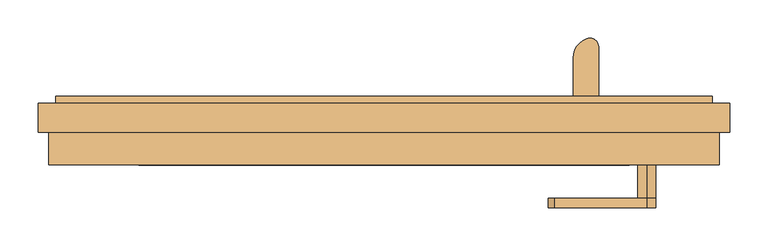
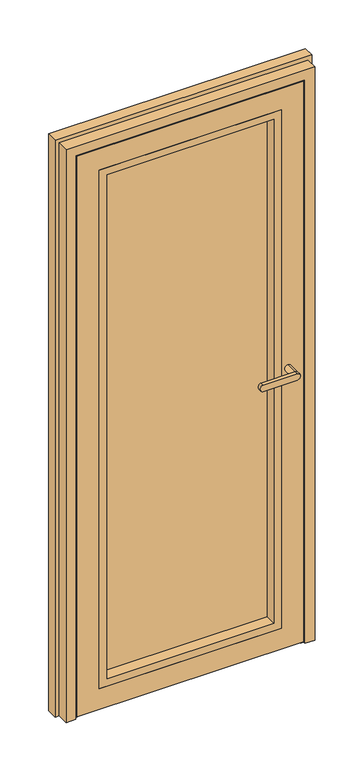
"""IFC4 building model written with IfcOpenShell, lengths in millimetres: door geometry, Schueco_FWS_ADS-90-SI_inw_Family-01 : FWS SI insert unit."""

from ifc_helpers import new_model, si_unit, point, frame, frame_2d, origin, place, context, project, spatial, polyline, circle_curve, ellipse_curve, trimmed, segment, composite_curve, outline, extrude, faceted_brep, source, transform, mapped, element, save
from ifc_brep_helpers import plane_surface, cylinder_surface, extruded_surface, advanced_brep


def door_b40c46e4(model_context):
    return source(origin(), model_context, "Body", "SolidModel", [
        extrude(outline(composite_curve([segment(polyline([(248.3327372, 8.9997177), (248.3327372, 59.1618682)]), True, "CONTINUOUS"), segment(trimmed(circle_curve(frame_2d((275.5111549, 59.1618682)), 27.1784177), [point((248.3327372, 59.1618682))], [point((265.9740593, 84.6120194))], False, "CARTESIAN"), True, "CONTINUOUS"), segment(trimmed(circle_curve(frame_2d((270.0515602, 73.7310321)), 11.6198924), [point((265.9740593, 84.6120194))], [point((281.6714526, 73.7310321))], False, "CARTESIAN"), True, "CONTINUOUS"), segment(polyline([(281.6714526, 73.7310321), (281.6714526, 8.9997177), (248.3327372, 8.9997177)]), True, "CONTINUOUS")], self_intersect=False)), frame((0.0, 0.0, 2043.9340013), z_axis=(0.0, 0.0, 1.0), x_axis=(1.0, 0.0, 0.0)), (0.0, 0.0, 1.0), 4.0),
        extrude(outline(polyline([(248.3327372, 12.9997177), (281.6714526, 12.9997177), (281.6714526, 8.9997177), (248.3327372, 8.9997177), (248.3327372, 12.9997177)])), frame((0.0, 0.0, 2013.9340013), z_axis=(0.0, 0.0, 1.0), x_axis=(1.0, 0.0, 0.0)), (0.0, 0.0, 1.0), 30.0),
        extrude(outline(polyline([(248.3327372, 12.9997177), (281.6714526, 12.9997177), (281.6714526, 8.9997177), (248.3327372, 8.9997177), (248.3327372, 12.9997177)])), frame((0.0, 0.0, 56.9340013), z_axis=(0.0, 0.0, 1.0), x_axis=(1.0, 0.0, 0.0)), (0.0, 0.0, 1.0), 30.0),
        extrude(outline(composite_curve([segment(polyline([(248.3327372, 8.9997177), (248.3327372, 59.1618682)]), True, "CONTINUOUS"), segment(trimmed(circle_curve(frame_2d((275.5111549, 59.1618682)), 27.1784177), [point((248.3327372, 59.1618682))], [point((265.9740593, 84.6120194))], False, "CARTESIAN"), True, "CONTINUOUS"), segment(trimmed(circle_curve(frame_2d((270.0515602, 73.7310321)), 11.6198924), [point((265.9740593, 84.6120194))], [point((281.6714526, 73.7310321))], False, "CARTESIAN"), True, "CONTINUOUS"), segment(polyline([(281.6714526, 73.7310321), (281.6714526, 8.9997177), (248.3327372, 8.9997177)]), True, "CONTINUOUS")], self_intersect=False)), frame((0.0, 0.0, 52.9340013), z_axis=(0.0, 0.0, 1.0), x_axis=(1.0, 0.0, 0.0)), (0.0, 0.0, 1.0), 4.0),
        advanced_brep(
        [(277.7171368, 57.5977179, 2043.9340013), (252.2829847, 72.2821425, 2043.9340013), (277.7171368, 57.5977179, 56.9340013), (252.2829847, 72.2821425, 56.9340013)],
        [
            (0, 1, ellipse_curve(frame((265.0000608, 64.9399302, 2043.9340013), z_axis=(0.0, 0.0, 1.0), x_axis=(0.5000002582658957, 0.866025254674503, 0.0)), 21.5840887, 14.6844171)),
            (1, 0, ellipse_curve(frame((265.0000608, 64.9399302, 2043.9340013), z_axis=(0.0, 0.0, 1.0), x_axis=(0.5000002582658957, 0.866025254674503, 0.0)), 21.5840887, 14.6844171)),
            (2, 3, ellipse_curve(frame((265.0000608, 64.9399302, 56.9340013), z_axis=(0.0, 0.0, -1.0), x_axis=(-0.866025254674503, 0.5000002582658957, 0.0)), 14.6844171, 21.5840887)),
            (3, 2, ellipse_curve(frame((265.0000608, 64.9399302, 56.9340013), z_axis=(0.0, 0.0, -1.0), x_axis=(-0.866025254674503, 0.5000002582658957, 0.0)), 14.6844171, 21.5840887)),
            (0, 2),
            (3, 1),
        ],
        [
            plane_surface(frame((252.2829847, 72.2821425, 2043.9340013), z_axis=(0.0, 0.0, 1.0), x_axis=(0.5000002582658957, 0.866025254674503, 0.0))),
            plane_surface(frame((252.2829847, 72.2821425, 56.9340013), z_axis=(0.0, 0.0, -1.0), x_axis=(-0.5000002582658957, -0.866025254674503, 0.0))),
            extruded_surface(trimmed(ellipse_curve(frame((265.0000608, 64.9399302, 56.9340013), z_axis=(0.0, 0.0, -1.0), x_axis=(-0.866025254674503, 0.5000002582658957, 0.0)), 14.6844171, 21.5840887), [point((252.2829847, 72.2821425, 56.9340013))], [point((277.7171368, 57.5977179, 56.9340013))], True, "CARTESIAN"), (0.0, 0.0, -1987.0), 1987.0),
            extruded_surface(trimmed(ellipse_curve(frame((265.0000608, 64.9399302, 56.9340013), z_axis=(0.0, 0.0, -1.0), x_axis=(-0.866025254674503, 0.5000002582658957, 0.0)), 14.6844171, 21.5840887), [point((277.7171368, 57.5977179, 56.9340013))], [point((252.2829847, 72.2821425, 56.9340013))], True, "CARTESIAN"), (0.0, 0.0, -1987.0), 1987.0),
        ],
        [
            (0, [[1, 2]]),
            (1, [[3, 4]]),
            (2, [[5, -4, 6, -1]]),
            (3, [[-6, -3, -5, -2]]),
        ],
    ),
        advanced_brep(
        [(345.0000608, -137.0002518, 1038.0113692), (345.0000608, -137.0002518, 1061.9886308), (223.3382682, -137.0002518, 1061.9886308), (223.3382682, -137.0002518, 1038.0113692), (345.0000608, -124.5001648, 1061.9886308), (345.0000608, -124.5001648, 1038.0113692), (223.3382682, -124.5001648, 1038.0113692), (223.3382682, -124.5001648, 1061.9886308), (345.0000608, -81.0002823, 1038.0113692), (345.0000608, -81.0002823, 1061.9886308)],
        [
            (0, 1, circle_curve(frame((345.0000608, -137.0002518, 1050.0), z_axis=(0.0, -1.0, 0.0), x_axis=(0.0, 0.0, 1.0)), 11.9886308)),
            (1, 2),
            (2, 3, ellipse_curve(frame((223.3382682, -137.0002518, 1050.0), z_axis=(0.0, -1.0, 0.0), x_axis=(0.0, 0.0, -1.0)), 11.9886308, 7.9050795)),
            (3, 0),
            (4, 5, circle_curve(frame((345.0000608, -124.5001648, 1050.0), z_axis=(0.0, -1.0, 0.0), x_axis=(0.0, 0.0, 1.0)), 11.9886308)),
            (5, 6),
            (6, 7, ellipse_curve(frame((223.3382682, -124.5001648, 1050.0), z_axis=(0.0, 1.0, 0.0), x_axis=(0.0, 0.0, -1.0)), 11.9886308, 7.9050795)),
            (7, 4),
            (3, 6),
            (5, 0),
            (2, 7),
            (1, 4),
            (5, 4, circle_curve(frame((345.0000608, -124.5001648, 1050.0), z_axis=(0.0, -1.0, 0.0), x_axis=(0.0, 0.0, 1.0)), 11.9886308)),
            (8, 9, circle_curve(frame((345.0000608, -81.0002823, 1050.0), z_axis=(0.0, 1.0, 0.0), x_axis=(0.0, 0.0, 1.0)), 11.9886308)),
            (9, 8, circle_curve(frame((345.0000608, -81.0002823, 1050.0), z_axis=(0.0, 1.0, 0.0), x_axis=(0.0, 0.0, 1.0)), 11.9886308)),
            (8, 5),
            (4, 9),
        ],
        [
            plane_surface(frame((223.3382682, -137.0002518, 1038.0113692), z_axis=(0.0, -1.0, 0.0), x_axis=(-1.0, 0.0, 0.0))),
            plane_surface(frame((223.3382682, -124.5001648, 1038.0113692), z_axis=(0.0, 1.0, 0.0), x_axis=(1.0, 0.0, 0.0))),
            plane_surface(frame((345.0000608, -137.0002518, 1038.0113692), z_axis=(0.0, 0.0, -1.0), x_axis=(0.0, 1.0, 0.0))),
            extruded_surface(trimmed(ellipse_curve(frame((223.3382682, -124.5001648, 1050.0), z_axis=(0.0, 1.0, 0.0), x_axis=(0.0, 0.0, -1.0)), 11.9886308, 7.9050795), [point((223.3382682, -124.5001648, 1038.0113692))], [point((223.3382682, -124.5001648, 1061.9886308))], True, "CARTESIAN"), (0.0, 12.500086999999994, 0.0), 12.500086999999994),
            plane_surface(frame((223.3382682, -137.0002518, 1061.9886308), z_axis=(0.0, 0.0, 1.0), x_axis=(0.0, 1.0, 0.0))),
            cylinder_surface(frame((345.0000608, -124.5001648, 1050.0), z_axis=(0.0, -1.0, 0.0), x_axis=(0.0, 0.0, 1.0)), 11.9886308),
            plane_surface(frame((345.0000608, -81.0002823, 1061.9886308), z_axis=(0.0, 1.0, 0.0), x_axis=(-1.0, 0.0, 0.0))),
            cylinder_surface(frame((345.0000608, -81.0002823, 1050.0), z_axis=(0.0, -1.0, 0.0), x_axis=(0.0, 0.0, 1.0)), 11.9886308),
        ],
        [
            (0, [[1, 2, 3, 4]]),
            (1, [[5, 6, 7, 8]]),
            (2, [[9, -6, 10, -4]]),
            (3, [[11, -7, -9, -3]]),
            (4, [[12, -8, -11, -2]]),
            (5, [[-10, 13, -12, -1]]),
            (6, [[14, 15]]),
            (7, [[16, -5, 17, -14]]),
            (7, [[-17, -13, -16, -15]]),
        ],
    ),
        extrude(outline(polyline([(86.0, 322.0000608), (2022.0, 322.0000608), (2022.0, -321.9999392), (86.0, -321.9999392), (86.0, 322.0000608)]), holes=[polyline([(113.0, -294.9999392), (1995.0, -294.9999392), (1995.0, 295.0000608), (113.0, 295.0000608), (113.0, -294.9999392)])]), frame((0.0, -81.0002823, 0.0), z_axis=(0.0, 1.0, 0.0), x_axis=(0.0, 0.0, 1.0)), (0.0, 0.0, 1.0), 41.0000097),
        faceted_brep([(-399.9999392, -81.0002823, 2100.0), (-399.9999392, -72.5000065, 2100.0), (-399.9999392, -72.5000065, 8.0), (-399.9999392, -81.0002823, 8.0), (400.0000608, -72.5000065, 8.0), (400.0000608, -81.0002823, 8.0), (400.0000608, -72.5000065, 2100.0), (382.0000608, -72.5000065, 26.0), (382.0000608, -72.5000065, 2082.0), (-381.9999392, -72.5000065, 2082.0), (-381.9999392, -72.5000065, 26.0), (400.0000608, -81.0002823, 2100.0), (-321.9999392, -81.0002823, 86.0), (-321.9999392, -81.0002823, 2022.0), (322.0000608, -81.0002823, 2022.0), (322.0000608, -81.0002823, 86.0), (-321.9999392, -2.0002726, 2022.0), (-321.9999392, -2.0002726, 86.0), (322.0000608, -2.0002726, 86.0), (322.0000608, -2.0002726, 2022.0), (-296.9999392, -2.0002726, 111.0), (-296.9999392, -2.0002726, 1997.0), (297.0000608, -2.0002726, 1997.0), (297.0000608, -2.0002726, 111.0), (-296.9999392, 8.9997177, 1997.0), (-296.9999392, 8.9997177, 111.0), (297.0000608, 8.9997177, 111.0), (297.0000608, 8.9997177, 1997.0), (-369.9999392, 8.9997177, 38.0), (-369.9999392, 8.9997177, 2070.0), (370.0000608, 8.9997177, 2070.0), (370.0000608, 8.9997177, 38.0), (-369.9999392, 0.4997603, 2070.0), (-369.9999392, 0.4997603, 38.0), (370.0000608, 0.4997603, 38.0), (370.0000608, 0.4997603, 2070.0), (-381.9999392, 0.4997603, 26.0), (-381.9999392, 0.4997603, 2082.0), (382.0000608, 0.4997603, 2082.0), (382.0000608, 0.4997603, 26.0)], [[[0, 1, 2, 3]], [[3, 2, 4, 5]], [[2, 1, 6, 4], [7, 8, 9, 10]], [[5, 4, 6, 11]], [[5, 11, 0, 3], [12, 13, 14, 15]], [[16, 13, 12, 17]], [[17, 12, 15, 18]], [[18, 15, 14, 19]], [[18, 19, 16, 17], [20, 21, 22, 23]], [[24, 21, 20, 25]], [[25, 20, 23, 26]], [[26, 23, 22, 27]], [[28, 29, 30, 31], [26, 27, 24, 25]], [[32, 29, 28, 33]], [[33, 28, 31, 34]], [[34, 31, 30, 35]], [[36, 37, 38, 39], [34, 35, 32, 33]], [[9, 37, 36, 10]], [[10, 36, 39, 7]], [[7, 39, 38, 8]], [[11, 6, 1, 0]], [[19, 14, 13, 16]], [[27, 22, 21, 24]], [[35, 30, 29, 32]], [[8, 38, 37, 9]]]),
        extrude(outline(polyline([(322.0000608, -40.0002726), (-321.9999392, -40.0002726), (-321.9999392, -2.0002726), (322.0000608, -2.0002726), (322.0000608, -40.0002726)])), frame((0.0, 0.0, 86.0), z_axis=(0.0, 0.0, 1.0), x_axis=(1.0, 0.0, 0.0)), (0.0, 0.0, 1.0), 1936.0),
        extrude(outline(composite_curve([segment(trimmed(circle_curve(frame_2d((-31.496302, 20.1647327)), 20.1687817), [point((-20.8439358, 3.0385292))], [point((-42.1486683, 3.0385292))], False, "CARTESIAN"), True, "CONTINUOUS"), segment(polyline([(-42.1486683, 3.0385292), (-42.1486683, 26.0), (-20.8439358, 26.0), (-20.8439358, 3.0385292)]), True, "CONTINUOUS")], self_intersect=False)), frame((-369.9999392, 0.0, 0.0), z_axis=(1.0, 0.0, 0.0), x_axis=(0.0, 1.0, 0.0)), (0.0, 0.0, 1.0), 740.0),
        extrude(outline(polyline([(-369.9999392, 0.4997603), (-369.9999392, 8.9997177), (370.0000608, 8.9997177), (370.0000608, 0.4997603), (-369.9999392, 0.4997603)])), frame((0.0, 0.0, 8.0), z_axis=(0.0, 0.0, 1.0), x_axis=(1.0, 0.0, 0.0)), (0.0, 0.0, 1.0), 30.0),
        faceted_brep([(430.999943, 8.9997177, 2130.999943), (430.999943, 0.0, 2130.999943), (430.999943, 0.0, 0.0), (430.999943, 8.9997177, 0.0), (-454.0, 0.0, 0.0), (-454.0, 0.0, 2154.0), (454.0, 0.0, 2154.0), (454.0, 0.0, 0.0), (-430.999943, 0.0, 2130.999943), (-430.999943, 0.0, 0.0), (454.0, -38.0, 0.0), (440.0, -38.0, 0.0), (440.0, -81.0002823, 0.0), (404.9276063, -81.0002823, 0.0), (404.9276063, -72.5000065, 0.0), (393.0000155, -72.5000065, 0.0), (393.0000155, 0.4997603, 0.0), (374.9999888, 0.4997603, 0.0), (374.9999888, 8.9997177, 0.0), (-374.9999888, 8.9997177, 0.0), (-430.999943, 8.9997177, 0.0), (-430.999943, 8.9997177, 2130.999943), (374.9999888, 8.9997177, 2074.9999888), (-374.9999888, 8.9997177, 2074.9999888), (404.9276063, -81.0002823, 2104.9276063), (404.9276063, -72.5000065, 2104.9276063), (-404.9276063, -72.5000065, 0.0), (-393.0000155, -72.5000065, 0.0), (-393.0000155, -72.5000065, 2093.0000155), (393.0000155, -72.5000065, 2093.0000155), (-404.9276063, -72.5000065, 2104.9276063), (-440.0, -81.0002823, 0.0), (-404.9276063, -81.0002823, 0.0), (-404.9276063, -81.0002823, 2104.9276063), (440.0, -81.0002823, 2140.0), (-440.0, -81.0002823, 2140.0), (440.0, -38.0, 2140.0), (-454.0, -38.0, 0.0), (-440.0, -38.0, 0.0), (-440.0, -38.0, 2140.0), (454.0, -38.0, 2154.0), (-454.0, -38.0, 2154.0), (-374.9999888, 0.4997603, 0.0), (-393.0000155, 0.4997603, 0.0), (374.9999888, 0.4997603, 2074.9999888), (-374.9999888, 0.4997603, 2074.9999888), (393.0000155, 0.4997603, 2093.0000155), (-393.0000155, 0.4997603, 2093.0000155)], [[[0, 1, 2, 3]], [[4, 5, 6, 7, 2, 1, 8, 9]], [[3, 2, 7, 10, 11, 12, 13, 14, 15, 16, 17, 18]], [[19, 20, 21, 0, 3, 18, 22, 23]], [[24, 25, 14, 13]], [[26, 27, 28, 29, 15, 14, 25, 30]], [[31, 32, 33, 24, 13, 12, 34, 35]], [[34, 12, 11, 36]], [[37, 38, 39, 36, 11, 10, 40, 41]], [[4, 9, 20, 19, 42, 43, 27, 26, 32, 31, 38, 37]], [[20, 9, 8, 21]], [[18, 17, 44, 22]], [[42, 19, 23, 45]], [[32, 26, 30, 33]], [[31, 35, 39, 38]], [[4, 37, 41, 5]], [[6, 40, 10, 7]], [[43, 42, 45, 44, 17, 16, 46, 47]], [[16, 15, 29, 46]], [[27, 43, 47, 28]], [[21, 8, 1, 0]], [[33, 30, 25, 24]], [[35, 34, 36, 39]], [[23, 22, 44, 45]], [[5, 41, 40, 6]], [[47, 46, 29, 28]]]),
    ])


if __name__ == "__main__":
    model = new_model("IFC4")
    model_context = context("Model", 3, world=origin())
    ifc_project = project(units=[si_unit("LENGTHUNIT", "METRE", prefix="MILLI")], contexts=[model_context])
    site = spatial("IfcSite", under=ifc_project)
    building = spatial("IfcBuilding", under=site)
    placement = place(None, origin())
    door_shape = door_b40c46e4(model_context)
    element("IfcDoor", 1, ObjectType="Schueco_FWS_ADS-90-SI_inw_Family-01 : FWS SI insert unit", at=placement, inside=building, context=model_context, shape_type="MappedRepresentation", body=[
        mapped(door_shape, transform((0.0, 0.0, 0.0), x_axis=(1.0, 0.0, 0.0), y_axis=(0.0, 1.0, 0.0), z_axis=(0.0, 0.0, 1.0))),
    ])
    save(model, "model.ifc")

# Revit data of these elements
# Type "Schueco_FWS_ADS-90-SI_inw_Family-01 : FWS SI insert unit"
#   Type Mark = "35"
#   __NOTE__ = "Data describes the optimum values of the entire system. The properites of a selected design option have to be determined on an individual basis!"
#   Wind load resistance = "Class C3"
#   Watertightness = "Class 7A"
#   Thermal insulation = "Uf = 1.2 W/(m²K)"
#   Sound insulation = "..."
#   Schueco thermal insulation standard = "Highly thermally insulated"
#   Opening type = "Inward-opening, Flush-fitted"
#   Model = "Schueco ADS 90.SI"
#   Mechanical loading = "Class 3"
#   Maximum leaf width in mm = "1400"
#   Maximum leaf weight in kg = "160"
#   Maximum leaf height in mm = "2500"
#   Material = "Aluminium"
#   Construction Type = "Door, single-leaf, inward-opening"
#   Manufacturer = "Schueco International KG"
#   Long term functionality = "..."
#   Glazing data = "Triple glazing 38mm"
#   Façade insert unit = "yes"
#   Family creation date = "08.2017"
#   Description = "Schueco Aluminium Door System (ADS)"
#   Burglar resistance = "Class RC 3"
#   Areas of use = "Public buildings, Side entrance"
#   Analytic Construction = "<None>"
#   Air permeability = "Class 4"
#   Width [instance default] = 1006.111 mm
#   Leaf opening angle [instance default] = 0.00°
#   IOf_T = 38 mm
#   Height [instance default] = 2012.289 mm
#   Glazing area [instance default] = 1.20724 m²
#   Distance from bottom to handles [instance default] = 1050 mm
#   Clear opening width [instance default] = 848.111 mm
#   Standard threshold = no
#   Low level threshold = yes
#   Handles = yes
#   Glass = none
#   Frame = Alu
#   Fittings = none
# Element 1 (IfcDoor, "Schueco_FWS_ADS-90-SI_inw_Family-01 : FWS SI insert unit")
#   Width = 908 mm
#   Height = 2154 mm
#   Glazing area = 1.12028 m²
#   Clear opening width = 750 mm
#   Materials on its faces: "Alu", "Glass"
# Materials
#   "Alu": class "Glas", colour RGB 140 140 140, transparency 0
#   "Glass": class "Glass", colour RGB 128 128 255, transparency 0.75, Description = "Soda Lime Glass", Cost = 0
